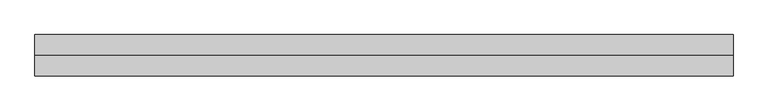
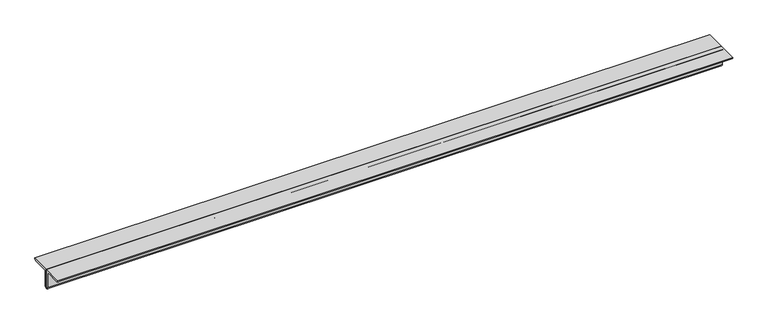
"""IFC4 building model written with IfcOpenShell, lengths in millimetres: member geometry, 0123_Steel Framing_2Ls-KSD3502 : H_SB_AR_S03_2Ls-130x130x12_HBR1."""

from ifc_helpers import new_model, si_unit, point, frame, frame_2d, origin, place, context, project, spatial, polyline, circle_curve, trimmed, segment, composite_curve, outline, extrude, source, transform, mapped, element, save


def member_7e9a97ce(model_context):
    return source(origin(), model_context, "Body", "SweptSolid", [
        extrude(outline(composite_curve([segment(polyline([(0.0, 36.4), (0.0, -93.6)]), True, "CONTINUOUS"), segment(trimmed(circle_curve(frame_2d((0.0, -81.6)), 12.0), [point((0.0, -93.6))], [point((-12.0, -81.6))], False, "CARTESIAN"), True, "CONTINUOUS"), segment(polyline([(-12.0, -81.6), (-12.0, 12.4)]), True, "CONTINUOUS"), segment(trimmed(circle_curve(frame_2d((-24.0, 12.4)), 12.0), [point((-12.0, 12.4))], [point((-24.0, 24.4))], True, "CARTESIAN"), True, "CONTINUOUS"), segment(polyline([(-24.0, 24.4), (-118.0, 24.4)]), True, "CONTINUOUS"), segment(trimmed(circle_curve(frame_2d((-118.0, 36.4)), 12.0), [point((-118.0, 24.4))], [point((-130.0, 36.4))], False, "CARTESIAN"), True, "CONTINUOUS"), segment(polyline([(-130.0, 36.4), (0.0, 36.4)]), True, "CONTINUOUS")], self_intersect=False)), frame((-2158.4448527, 0.0, 0.0), z_axis=(1.0, 0.0, 0.0), x_axis=(0.0, 1.0, 0.0)), (0.0, 0.0, 1.0), 4391.0649986),
        extrude(outline(composite_curve([segment(polyline([(0.0, 36.4), (130.0, 36.4)]), True, "CONTINUOUS"), segment(trimmed(circle_curve(frame_2d((118.0, 36.4)), 12.0), [point((130.0, 36.4))], [point((118.0, 24.4))], False, "CARTESIAN"), True, "CONTINUOUS"), segment(polyline([(118.0, 24.4), (24.0, 24.4)]), True, "CONTINUOUS"), segment(trimmed(circle_curve(frame_2d((24.0, 12.4)), 12.0), [point((24.0, 24.4))], [point((12.0, 12.4))], True, "CARTESIAN"), True, "CONTINUOUS"), segment(polyline([(12.0, 12.4), (12.0, -81.6)]), True, "CONTINUOUS"), segment(trimmed(circle_curve(frame_2d((0.0, -81.6)), 12.0), [point((12.0, -81.6))], [point((0.0, -93.6))], False, "CARTESIAN"), True, "CONTINUOUS"), segment(polyline([(0.0, -93.6), (0.0, 36.4)]), True, "CONTINUOUS")], self_intersect=False)), frame((-2158.4448527, 0.0, 0.0), z_axis=(1.0, 0.0, 0.0), x_axis=(0.0, 1.0, 0.0)), (0.0, 0.0, 1.0), 4391.0649986),
    ])


if __name__ == "__main__":
    model = new_model("IFC4")
    model_context = context("Model", 3, world=origin())
    ifc_project = project(units=[si_unit("LENGTHUNIT", "METRE", prefix="MILLI")], contexts=[model_context])
    site = spatial("IfcSite", under=ifc_project)
    building = spatial("IfcBuilding", under=site)
    placement = place(None, origin())
    member_shape = member_7e9a97ce(model_context)
    element("IfcMember", 1, ObjectType="0123_Steel Framing_2Ls-KSD3502 : H_SB_AR_S03_2Ls-130x130x12_HBR1", at=placement, inside=building, context=model_context, shape_type="MappedRepresentation", body=[
        mapped(member_shape, transform((0.0, 0.0, 0.0), x_axis=(1.0, 0.0, 0.0), y_axis=(0.0, 1.0, 0.0), z_axis=(0.0, 0.0, 1.0))),
    ])
    save(model, "model.ifc")

# Revit data of these elements
# Type "0123_Steel Framing_2Ls-KSD3502 : H_SB_AR_S03_2Ls-130x130x12_HBR1"
#   Type Mark = "HBR1"
#   Assembly Code = "B10"
#   Legs = "SLBB"
#   W = 8.97
#   Perimeter = 1.04 m²/m
#   Nominal Weight = 46.80 kgf/m
#   Length [instance default] = 1000 mm
#   Space = 0 mm
#   b = 130 mm
#   d = 130 mm
#   t = 12 mm
#   y = 36.4 mm
#   A = 0.005952 m²
#   Structural Material [instance default] = Steel ASTM A36
# Element 1 (IfcMember, "0123_Steel Framing_2Ls-KSD3502 : H_SB_AR_S03_2Ls-130x130x12_HBR1")
#   Materials on its faces: "Steel ASTM A36"
# Materials
#   "Steel ASTM A36": class "Metal", colour RGB 199 199 199, transparency 0, Description = "Structural steel, ASTM A36 Grade B, mill finish", Cost = 0
